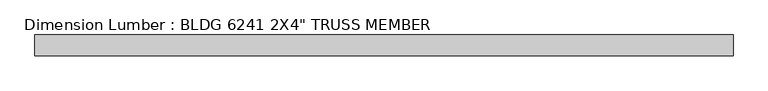
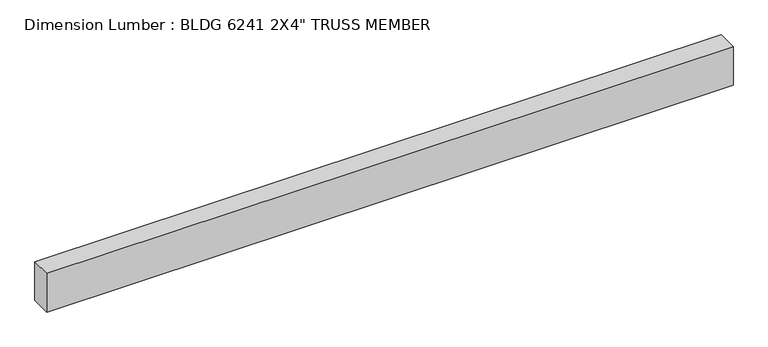
"""IFC4 building model written with IfcOpenShell, lengths in millimetres: beam geometry."""

from ifc_helpers import new_model, si_unit, frame, origin, place, context, project, spatial, polyline, outline, extrude, source, transform, mapped, element, save


def beam_3500c81b(model_context):
    return source(origin(), model_context, "Body", "SweptSolid", [
        extrude(outline(polyline([(863.6, 25.4), (863.6, -25.4), (-845.1882072, -25.4), (-845.1882072, 25.4), (863.6, 25.4)])), frame((0.0, 0.0, -50.8), z_axis=(0.0, 0.0, 1.0), x_axis=(1.0, 0.0, 0.0)), (0.0, 0.0, 1.0), 101.6),
    ])


if __name__ == "__main__":
    model = new_model("IFC4")
    model_context = context("Model", 3, world=origin())
    ifc_project = project(units=[si_unit("LENGTHUNIT", "METRE", prefix="MILLI")], contexts=[model_context])
    site = spatial("IfcSite", under=ifc_project)
    building = spatial("IfcBuilding", under=site)
    placement = place(None, origin())
    beam_shape = beam_3500c81b(model_context)
    element("IfcBeam", 1, ObjectType="Dimension Lumber : BLDG 6241 2X4\" TRUSS MEMBER", at=placement, inside=building, context=model_context, shape_type="MappedRepresentation", body=[
        mapped(beam_shape, transform((0.0, 0.0, 0.0), x_axis=(1.0, 0.0, 0.0), y_axis=(0.0, 1.0, 0.0), z_axis=(0.0, 0.0, 1.0))),
    ])
    save(model, "model.ifc")

# Revit data of these elements
# Type "Dimension Lumber : BLDG 6241 2X4\" TRUSS MEMBER"
#   Assembly Code = "B10"
#   A = 0.273472 SF
#   Length [instance default] = 5' - 0"
#   b = 0' - 2"
#   d = 0' - 4"
#   Structural Material [instance default] = Softwood, Lumber
# Element 1 (IfcBeam, "Dimension Lumber : BLDG 6241 2X4\" TRUSS MEMBER")
#   Materials on its faces: "Softwood, Lumber"
# Materials
#   "Softwood, Lumber": class "Wood", colour RGB 223 192 134, transparency 0, Description = "Pinus Echinata", Cost = 0
